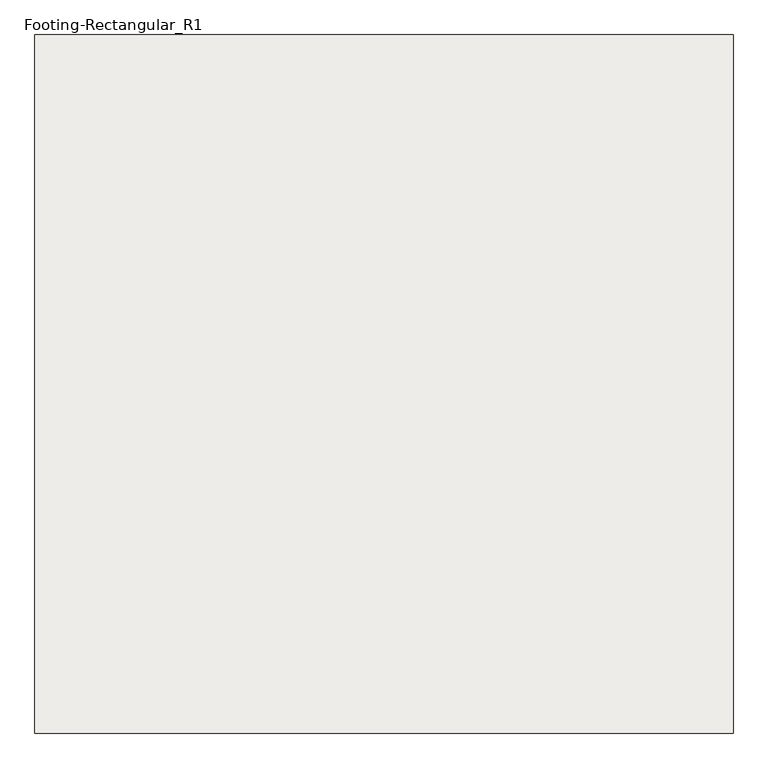
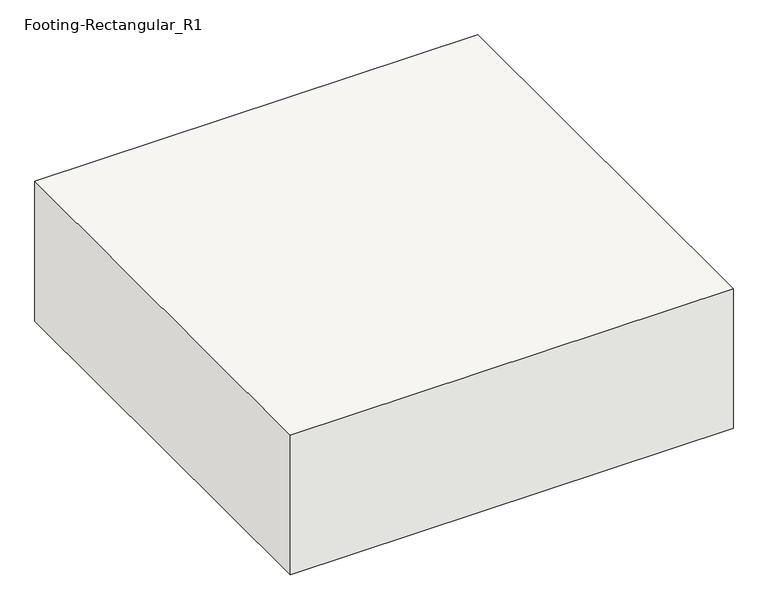
"""IFC4 building model written with IfcOpenShell, lengths in millimetres: slab geometry, Footing-Rectangular_R1 : H_SF_AR_S18_W1500xL1500xT500_Bitumen_F2."""

from ifc_helpers import new_model, si_unit, frame, origin, place, context, project, spatial, polyline, outline, extrude, source, transform, mapped, element, save


def footing_rectangular_r1_601d9235(model_context):
    return source(origin(), model_context, "Body", "SweptSolid", [
        extrude(outline(polyline([(750.0, 750.0), (750.0, -750.0), (-750.0, -750.0), (-750.0, 750.0), (750.0, 750.0)])), frame((0.0, 0.0, -500.0), z_axis=(0.0, 0.0, 1.0), x_axis=(1.0, 0.0, 0.0)), (0.0, 0.0, 1.0), 500.0),
    ])


if __name__ == "__main__":
    model = new_model("IFC4")
    model_context = context("Model", 3, world=origin())
    ifc_project = project(units=[si_unit("LENGTHUNIT", "METRE", prefix="MILLI")], contexts=[model_context])
    site = spatial("IfcSite", under=ifc_project)
    building = spatial("IfcBuilding", under=site)
    placement = place(None, origin())
    footing_rectangular_r1_shape = footing_rectangular_r1_601d9235(model_context)
    element("IfcSlab", 1, ObjectType="Footing-Rectangular_R1 : H_SF_AR_S18_W1500xL1500xT500_Bitumen_F2", at=placement, inside=building, context=model_context, shape_type="MappedRepresentation", body=[
        mapped(footing_rectangular_r1_shape, transform((0.0, 0.0, 0.0), x_axis=(1.0, 0.0, 0.0), y_axis=(0.0, 1.0, 0.0), z_axis=(0.0, 0.0, 1.0))),
    ])
    save(model, "model.ifc")

# Revit data of these elements
# Type "Footing-Rectangular_R1 : H_SF_AR_S18_W1500xL1500xT500_Bitumen_F2"
#   Type Mark = "F2"
#   Top bar = "D25@300"
#   Description = "UG Shallow Foundation"
#   Bottom bar = "D20@300"
#   Width = 1500 mm
#   Length = 1500 mm
#   Foundation Thickness = 500 mm
#   Structural Material [instance default] = none
#   Assembly Code = ""
